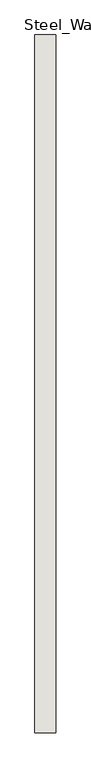
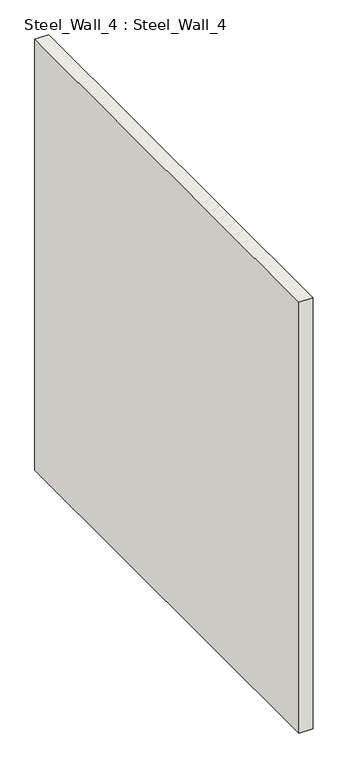
"""IFC4 building model written with IfcOpenShell, lengths in millimetres: wall geometry, Steel_Wall_4 : Steel_Wall_4."""

from ifc_helpers import new_model, si_unit, frame, origin, place, context, project, spatial, polyline, outline, extrude, source, transform, mapped, element, save


def steel_wall_4_steel_wall_4_2983a264(model_context):
    return source(origin(), model_context, "Body", "SweptSolid", [
        extrude(outline(polyline([(215.0, 15685.0), (215.0, 12365.0), (115.0, 12365.0), (115.0, 15685.0), (215.0, 15685.0)])), frame((0.0, 0.0, 250.0), z_axis=(0.0, 0.0, 1.0), x_axis=(1.0, 0.0, 0.0)), (0.0, 0.0, 1.0), 3300.0),
    ])


if __name__ == "__main__":
    model = new_model("IFC4")
    model_context = context("Model", 3, world=origin())
    ifc_project = project(units=[si_unit("LENGTHUNIT", "METRE", prefix="MILLI")], contexts=[model_context])
    site = spatial("IfcSite", under=ifc_project)
    building = spatial("IfcBuilding", under=site)
    placement = place(None, origin())
    steel_wall_4_steel_wall_4_shape = steel_wall_4_steel_wall_4_2983a264(model_context)
    element("IfcWall", 1, ObjectType="Steel_Wall_4 : Steel_Wall_4", at=placement, inside=building, context=model_context, shape_type="MappedRepresentation", body=[
        mapped(steel_wall_4_steel_wall_4_shape, transform((0.0, 0.0, 0.0), x_axis=(1.0, 0.0, 0.0), y_axis=(0.0, 1.0, 0.0), z_axis=(0.0, 0.0, 1.0))),
    ])
    save(model, "model.ifc")

# Revit data of these elements
# Type "Steel_Wall_4 : Steel_Wall_4"
#   NameOverride = "Steel_Wall_4"
# Element 1 (IfcWall, "Steel_Wall_4 : Steel_Wall_4")
#   Materials on its faces: "IfcSurfaceStyle #33"
# Materials
#   "IfcSurfaceStyle #33": class "Unassigned", colour RGB 214 214 214, transparency 0
